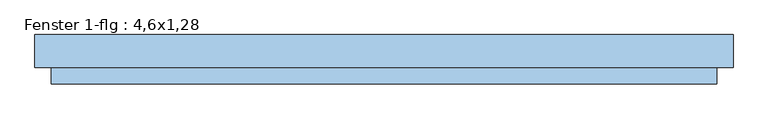
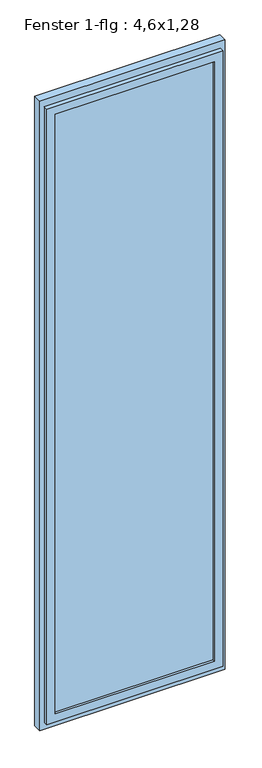
"""IFC4 building model written with IfcOpenShell, lengths in millimetres: window geometry, Fenster 1-flg : 4,6x1,28."""

from ifc_helpers import new_model, si_unit, frame, origin, place, context, project, spatial, polyline, outline, extrude, faceted_brep, source, transform, mapped, element, save


def fenster_1_flg_4_6x1_28_cf6fbe01(model_context):
    return source(origin(), model_context, "Body", "SolidModel", [
        extrude(outline(polyline([(5600.0, 640.0), (5600.0, -640.0), (1000.0, -640.0), (1000.0, 640.0), (5600.0, 640.0)]), holes=[polyline([(5520.0, 580.0), (1080.0, 580.0), (1080.0, -580.0), (5520.0, -580.0), (5520.0, 580.0)])]), frame((0.0, 20.0, 0.0), z_axis=(0.0, 1.0, 0.0), x_axis=(0.0, 0.0, 1.0)), (0.0, 0.0, 1.0), 60.0),
        faceted_brep([(610.0, 20.0, 5550.0), (610.0, -10.0, 5550.0), (610.0, -10.0, 1050.0), (610.0, 20.0, 1050.0), (-610.0, -10.0, 5550.0), (-610.0, -10.0, 1050.0), (550.0, -10.0, 1110.0), (-550.0, -10.0, 1110.0), (-550.0, -10.0, 5490.0), (550.0, -10.0, 5490.0), (-610.0, 20.0, 1050.0), (-610.0, 20.0, 5550.0), (580.0, 20.0, 5520.0), (-580.0, 20.0, 5520.0), (-580.0, 20.0, 1080.0), (580.0, 20.0, 1080.0), (580.0, 50.0, 5520.0), (580.0, 50.0, 1080.0), (-580.0, 50.0, 1080.0), (-580.0, 50.0, 5520.0), (550.0, 50.0, 5490.0), (-550.0, 50.0, 5490.0), (-550.0, 50.0, 1110.0), (550.0, 50.0, 1110.0)], [[[0, 1, 2, 3]], [[1, 4, 5, 2], [6, 7, 8, 9]], [[3, 2, 5, 10]], [[3, 10, 11, 0], [12, 13, 14, 15]], [[16, 12, 15, 17]], [[17, 15, 14, 18]], [[17, 18, 19, 16], [20, 21, 22, 23]], [[9, 20, 23, 6]], [[6, 23, 22, 7]], [[10, 5, 4, 11]], [[18, 14, 13, 19]], [[7, 22, 21, 8]], [[11, 4, 1, 0]], [[19, 13, 12, 16]], [[8, 21, 20, 9]]]),
        extrude(outline(polyline([(550.0, 5.0), (-550.0, 5.0), (-550.0, 35.0), (550.0, 35.0), (550.0, 5.0)])), frame((0.0, 0.0, 1110.0), z_axis=(0.0, 0.0, 1.0), x_axis=(1.0, 0.0, 0.0)), (0.0, 0.0, 1.0), 4380.0),
    ])


if __name__ == "__main__":
    model = new_model("IFC4")
    model_context = context("Model", 3, world=origin())
    ifc_project = project(units=[si_unit("LENGTHUNIT", "METRE", prefix="MILLI")], contexts=[model_context])
    site = spatial("IfcSite", under=ifc_project)
    building = spatial("IfcBuilding", under=site)
    placement = place(None, origin())
    fenster_1_flg_4_6x1_28_shape = fenster_1_flg_4_6x1_28_cf6fbe01(model_context)
    element("IfcWindow", 1, ObjectType="Fenster 1-flg : 4,6x1,28", at=placement, inside=building, context=model_context, shape_type="MappedRepresentation", body=[
        mapped(fenster_1_flg_4_6x1_28_shape, transform((0.0, 0.0, 0.0), x_axis=(1.0, 0.0, 0.0), y_axis=(0.0, 1.0, 0.0), z_axis=(0.0, 0.0, 1.0))),
    ])
    save(model, "model.ifc")

# Revit data of these elements
# Type "Fenster 1-flg : 4,6x1,28"
#   Type Mark = "67"
#   Operation = "SinglePanel"
#   Keynote = "16.05.01"
#   Visual Light Transmittance = 0.9
#   Solar Heat Gain Coefficient = 0.86
#   Rough Width = 1.280 m
#   Rough Height = 4.600 m
#   Heat Transfer Coefficient (U) = 5.5617 W/(m²·K)
#   Rahmentiefe = 0.060 m
#   Rahmenhöhe - unten = 0.080 m
#   Rahmenhöhe - oben = 0.080 m
#   Rahmenbreite = 0.060 m
#   Height = 4.600 m
#   Tiefe Flügel = 0.060 m
#   Flügelbreite = 0.060 m
#   Einbautiefe (von außen) [instance default] = 0.100 m
#   Width = 1.280 m
#   Klappflügel [instance default] = no
#   Kippflügel [instance default] = yes
#   Öffnungsrichtung in Draufsicht anzeigen [instance default] = no
#   Drehflügel 1 [instance default] = yes
#   Rahmen 1 [instance default] = none
#   Glas [instance default] = none
#   Flügel [instance default] = none
#   Fensterbank Innenseite [instance default] = none
#   Fensterbank Außenseite [instance default] = none
#   Construction Type Id = ""
#   Wall Closure = (empty or 0)
#   Analytic Construction = (empty or 0)
# Element 1 (IfcWindow, "Fenster 1-flg : 4,6x1,28")
#   Einbautiefe (von außen) = 0.230 m
#   Materials on its faces: "Kunststoff - Weiß", "Glas"
# Materials
#   "Kunststoff - Weiß": class "Kunststoff", colour RGB 249 249 249, transparency 0, Cost = 0
#   "Glas": class "Glas", colour RGB 0 0 255, transparency 0.75, Comments = "Render-Darstellung nicht aktualisiert ", Cost = 0
